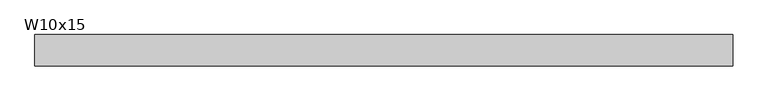
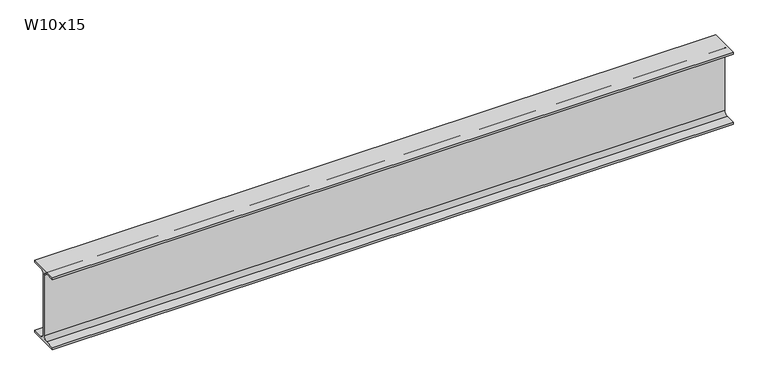
"""IFC4 building model written with IfcOpenShell, lengths in millimetres: beam geometry, RME W-Wide Flange : W10x15."""

from ifc_helpers import new_model, si_unit, point, frame, frame_2d, origin, place, context, project, spatial, polyline, circle_curve, trimmed, segment, composite_curve, outline, extrude, source, transform, mapped, element, save


def w10x15_dbc2b807(model_context):
    return source(origin(), model_context, "Body", "SweptSolid", [
        extrude(outline(composite_curve([segment(polyline([(50.8, -120.142), (50.8, -127.0), (-50.8, -127.0), (-50.8, -120.142), (-16.7005, -120.142)]), True, "CONTINUOUS"), segment(trimmed(circle_curve(frame_2d((-16.7005, -106.3625)), 13.7795), [point((-16.7005, -120.142))], [point((-2.921, -106.3625))], True, "CARTESIAN"), True, "CONTINUOUS"), segment(polyline([(-2.921, -106.3625), (-2.921, 106.3625)]), True, "CONTINUOUS"), segment(trimmed(circle_curve(frame_2d((-16.7005, 106.3625)), 13.7795), [point((-2.921, 106.3625))], [point((-16.7005, 120.142))], True, "CARTESIAN"), True, "CONTINUOUS"), segment(polyline([(-16.7005, 120.142), (-50.8, 120.142), (-50.8, 127.0), (50.8, 127.0), (50.8, 120.142), (16.7005, 120.142)]), True, "CONTINUOUS"), segment(trimmed(circle_curve(frame_2d((16.7005, 106.3625)), 13.7795), [point((16.7005, 120.142))], [point((2.921, 106.3625))], True, "CARTESIAN"), True, "CONTINUOUS"), segment(polyline([(2.921, 106.3625), (2.921, -106.3625)]), True, "CONTINUOUS"), segment(trimmed(circle_curve(frame_2d((16.7005, -106.3625)), 13.7795), [point((2.921, -106.3625))], [point((16.7005, -120.142))], True, "CARTESIAN"), True, "CONTINUOUS"), segment(polyline([(16.7005, -120.142), (50.8, -120.142)]), True, "CONTINUOUS")], self_intersect=False)), frame((-1143.0, 0.0, 0.0), z_axis=(1.0, 0.0, 0.0), x_axis=(0.0, 1.0, 0.0)), (0.0, 0.0, 1.0), 2273.2999994),
    ])


if __name__ == "__main__":
    model = new_model("IFC4")
    model_context = context("Model", 3, world=origin())
    ifc_project = project(units=[si_unit("LENGTHUNIT", "METRE", prefix="MILLI")], contexts=[model_context])
    site = spatial("IfcSite", under=ifc_project)
    building = spatial("IfcBuilding", under=site)
    placement = place(None, origin())
    w10x15_shape = w10x15_dbc2b807(model_context)
    element("IfcBeam", 1, ObjectType="RME W-Wide Flange : W10x15", at=placement, inside=building, context=model_context, shape_type="MappedRepresentation", body=[
        mapped(w10x15_shape, transform((0.0, 0.0, 0.0), x_axis=(1.0, 0.0, 0.0), y_axis=(0.0, 1.0, 0.0), z_axis=(0.0, 0.0, 1.0))),
    ])
    save(model, "model.ifc")

# Revit data of these elements
# Type "RME W-Wide Flange : W10x15"
#   WELD P [instance default] = ""
#   WELD LE [instance default] = ""
#   WELD D [instance default] = ""
#   TOP SECTION SIZE [instance default] = ""
#   TOP SECTION LENGTH [instance default] = ""
#   REMARKS [instance default] = ""
#   REINF TYPE [instance default] = ""
#   Nominal Size = "W24"
#   End Bearing Capacity [instance default] = ""
#   BOT SECTION SIZE [instance default] = ""
#   BOT SECTION LENGTH [instance default] = ""
#   Assembly Code = "B10"
#   W = 15
#   Start Extension Calculation [instance default] = 10' - 0"
#   Start Extension [instance default] = -0' - 0 1/2"
#   End Extension Calculation [instance default] = 10' - 0"
#   End Extension [instance default] = -0' - 0 1/2"
#   Length [instance default] = 5' - 0"
#   bf = 0' - 4"
#   d = 0' - 10"
#   k = 0' - 0 13/16"
#   k2 = 0' - 0.5425"
#   tf = 0' - 0.27"
#   tw = 0' - 0.23"
#   A = 0.030625 SF
#   Structural Material [instance default] = Metal - Steel - ASTM A992
# Element 1 (IfcBeam, "RME W-Wide Flange : W10x15")
#   Length = 7' - 6"
#   Materials on its faces: "Metal - Steel - ASTM A992"
# Materials
#   "Metal - Steel - ASTM A992": class "Metal", colour RGB 255 128 0, transparency 0
